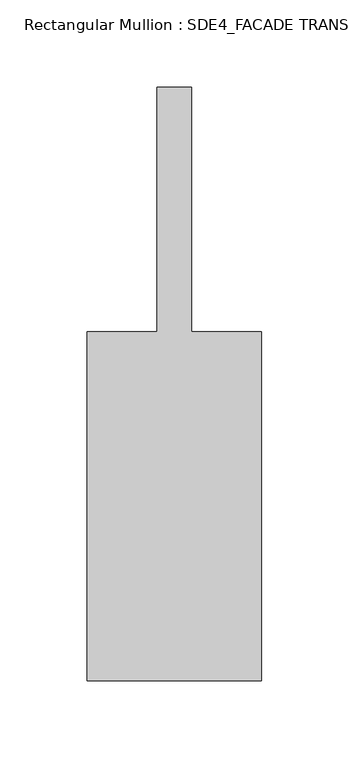
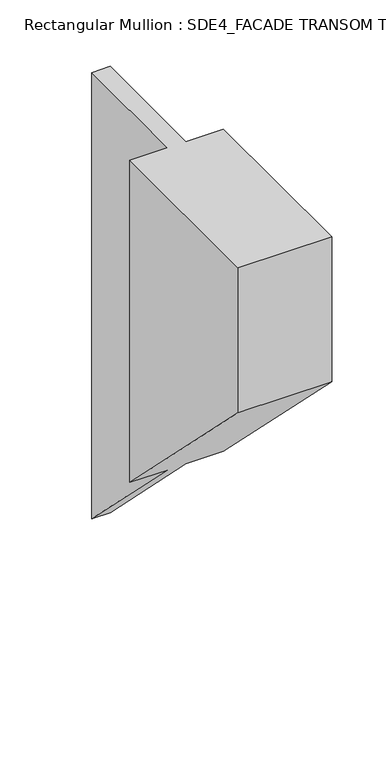
"""IFC4 building model written with IfcOpenShell, lengths in millimetres: member geometry, Rectangular Mullion : SDE4_FACADE TRANSOM TYPE 1."""

from ifc_helpers import new_model, si_unit, origin, place, context, project, spatial, faceted_brep, source, transform, mapped, element, save


def rectangular_mullion_sde4_facade_transom_type_1_760f2cdd(model_context):
    return source(origin(), model_context, "Body", "Brep", [
        faceted_brep([(50.0, -132.5, 0.0), (50.0, 67.5, 0.0), (10.0, 67.5, 0.0), (10.0, 207.5, 0.0), (-10.0, 207.5, 0.0), (-10.0, 67.5, 0.0), (-50.0, 67.5, 0.0), (-50.0, -132.5, 0.0), (50.0, -132.5, -163.7014804), (50.0, 67.5, -363.7014804), (10.0, 67.5, -363.7014804), (10.0, 207.5, -503.7014804), (-10.0, 207.5, -503.7014804), (-10.0, 67.5, -363.7014804), (-50.0, 67.5, -363.7014804), (-50.0, -132.5, -163.7014804)], [[[0, 1, 2, 3, 4, 5, 6, 7]], [[1, 0, 8, 9]], [[2, 1, 9, 10]], [[3, 2, 10, 11]], [[4, 3, 11, 12]], [[5, 4, 12, 13]], [[6, 5, 13, 14]], [[7, 6, 14, 15]], [[0, 7, 15, 8]], [[8, 15, 14, 13, 12, 11, 10, 9]]]),
    ])


if __name__ == "__main__":
    model = new_model("IFC4")
    model_context = context("Model", 3, world=origin())
    ifc_project = project(units=[si_unit("LENGTHUNIT", "METRE", prefix="MILLI")], contexts=[model_context])
    site = spatial("IfcSite", under=ifc_project)
    building = spatial("IfcBuilding", under=site)
    placement = place(None, origin())
    rectangular_mullion_sde4_facade_transom_type_1_shape = rectangular_mullion_sde4_facade_transom_type_1_760f2cdd(model_context)
    element("IfcMember", 1, ObjectType="Rectangular Mullion : SDE4_FACADE TRANSOM TYPE 1", at=placement, inside=building, context=model_context, shape_type="MappedRepresentation", body=[
        mapped(rectangular_mullion_sde4_facade_transom_type_1_shape, transform((0.0, 0.0, 0.0), x_axis=(1.0, 0.0, 0.0), y_axis=(0.0, 1.0, 0.0), z_axis=(0.0, 0.0, 1.0))),
    ])
    save(model, "model.ifc")

# Revit data of these elements
# Type "Rectangular Mullion : SDE4_FACADE TRANSOM TYPE 1"
#   built-in parameter 1007322 = 1.11549 (stored number, unit not read)
#   built-in parameter 1007321 = 0.164042 (stored number, unit not read)
#   built-in parameter 1007320 = 0.164042 (stored number, unit not read)
